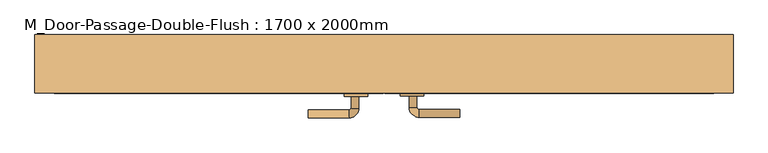
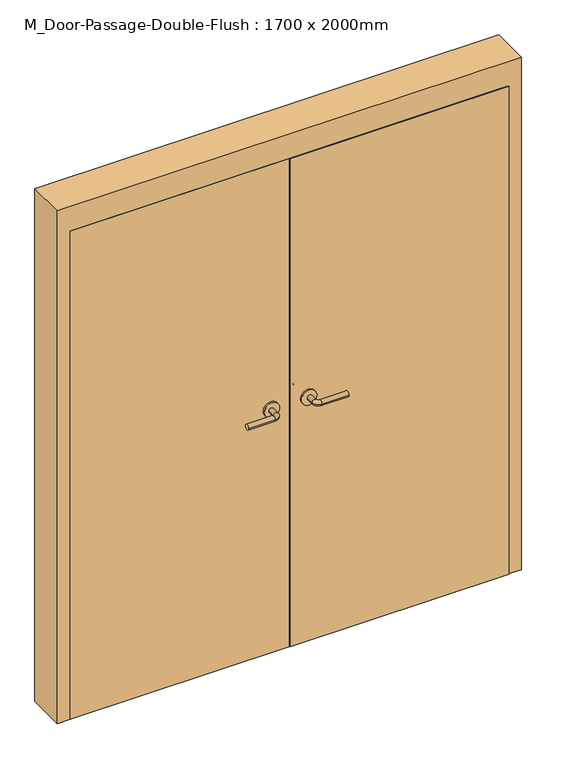
"""IFC4 building model written with IfcOpenShell, lengths in millimetres: door geometry, M_Door-Passage-Double-Flush : 1700 x 2000mm."""

from ifc_helpers import new_model, si_unit, point, frame, frame_2d, origin, origin_with_axes, place, context, project, spatial, polyline, circle_curve, ellipse_curve, trimmed, segment, composite_curve, outline, extrude, faceted_brep, source, transform, mapped, element, save
from ifc_brep_helpers import plane_surface, cylinder_surface, revolved_surface, advanced_brep


def m_door_passage_double_flush_1700_x_2000mm_96374c9b(model_context):
    return source(origin(), model_context, "Body", "SolidModel", [
        advanced_brep(
        [(-65.009375, -28.35, 1016.0), (-85.009375, -28.35, 1016.0), (-85.009375, 1.65, 1016.0), (-65.009375, 1.65, 1016.0), (-90.009375, 6.65, 1016.0), (-90.009375, 26.65, 1016.0), (-195.009375, 26.65, 1016.0), (-195.009375, 6.65, 1016.0)],
        [
            (0, 1, circle_curve(frame((-75.009375, -28.35, 1016.0), z_axis=(0.0, -1.0, 0.0), x_axis=(-1.0, 0.0, 0.0)), 10.0)),
            (1, 0, circle_curve(frame((-75.009375, -28.35, 1016.0), z_axis=(0.0, -1.0, 0.0), x_axis=(-1.0, 0.0, 0.0)), 10.0)),
            (1, 2),
            (2, 3, circle_curve(frame((-75.009375, 1.65, 1016.0), z_axis=(0.0, -1.0, 0.0), x_axis=(-1.0, 0.0, 0.0)), 10.0)),
            (3, 0),
            (3, 2, circle_curve(frame((-75.009375, 1.65, 1016.0), z_axis=(0.0, -1.0, 0.0), x_axis=(-1.0, 0.0, 0.0)), 10.0)),
            (4, 5, circle_curve(frame((-90.009375, 16.65, 1016.0), z_axis=(1.0, 0.0, 0.0), x_axis=(0.0, -1.0, 0.0)), 10.0)),
            (5, 3, circle_curve(frame((-90.009375, 1.65, 1016.0), z_axis=(0.0, 0.0, -1.0), x_axis=(1.0, 0.0, 0.0)), 25.0)),
            (2, 4, circle_curve(frame((-90.009375, 1.65, 1016.0), z_axis=(0.0, 0.0, 1.0), x_axis=(1.0, 0.0, 0.0)), 5.0)),
            (5, 4, circle_curve(frame((-90.009375, 16.65, 1016.0), z_axis=(1.0, 0.0, 0.0), x_axis=(0.0, -1.0, 0.0)), 10.0)),
            (6, 7, circle_curve(frame((-195.009375, 16.65, 1016.0), z_axis=(-1.0, 0.0, 0.0), x_axis=(0.0, -1.0, 0.0)), 10.0)),
            (7, 6, circle_curve(frame((-195.009375, 16.65, 1016.0), z_axis=(-1.0, 0.0, 0.0), x_axis=(0.0, -1.0, 0.0)), 10.0)),
            (4, 7),
            (6, 5),
        ],
        [
            plane_surface(frame((-75.009375, -28.35, 1016.0), z_axis=(0.0, -1.0, 0.0), x_axis=(0.0, 0.0, 1.0))),
            cylinder_surface(frame((-75.009375, -28.35, 1016.0), z_axis=(0.0, -1.0, 0.0), x_axis=(-1.0, 0.0, 0.0)), 10.0),
            revolved_surface(trimmed(ellipse_curve(frame((-75.009375, 1.65, 1016.0), z_axis=(0.0, 1.0, 0.0), x_axis=(-1.0, 0.0, 0.0)), 10.0, 10.0), [point((-65.009375, 1.65, 1016.0))], [point((-85.009375, 1.65, 1016.0))], True, "CARTESIAN"), (-90.009375, 1.65, 1016.0), (0.0, 0.0, -1.0)),
            revolved_surface(trimmed(ellipse_curve(frame((-75.009375, 1.65, 1016.0), z_axis=(0.0, 1.0, 0.0), x_axis=(-1.0, 0.0, 0.0)), 10.0, 10.0), [point((-85.009375, 1.65, 1016.0))], [point((-65.009375, 1.65, 1016.0))], True, "CARTESIAN"), (-90.009375, 1.65, 1016.0), (0.0, 0.0, -1.0)),
            plane_surface(frame((-195.009375, 16.65, 1016.0), z_axis=(-1.0, 0.0, 0.0), x_axis=(0.0, 0.0, 1.0))),
            cylinder_surface(frame((-90.009375, 16.65, 1016.0), z_axis=(1.0, 0.0, 0.0), x_axis=(0.0, -1.0, 0.0)), 10.0),
        ],
        [
            (0, [[1, 2]]),
            (1, [[3, 4, 5, -2]]),
            (1, [[-5, 6, -3, -1]]),
            (2, [[7, 8, -4, 9]]),
            (3, [[10, -9, -6, -8]]),
            (4, [[11, 12]]),
            (5, [[13, -11, 14, -7]]),
            (5, [[-14, -12, -13, -10]]),
        ],
    ),
        extrude(outline(composite_curve([segment(trimmed(circle_curve(frame_2d((1016.0, -72.509375)), 30.0), [point((1016.0, -42.509375))], [point((1016.0, -102.509375))], False, "CARTESIAN"), True, "CONTINUOUS"), segment(trimmed(circle_curve(frame_2d((1016.0, -72.509375)), 30.0), [point((1016.0, -102.509375))], [point((1016.0, -42.509375))], False, "CARTESIAN"), True, "CONTINUOUS")], self_intersect=False)), frame((0.0, -36.35, 0.0), z_axis=(0.0, 1.0, 0.0), x_axis=(0.0, 0.0, 1.0)), (0.0, 0.0, 1.0), 8.0),
        advanced_brep(
        [(-65.009375, -90.95, 1000.0), (-85.009375, -90.95, 1000.0), (-65.009375, -120.95, 1000.0), (-85.009375, -120.95, 1000.0), (-90.009375, -125.95, 1000.0), (-90.009375, -145.95, 1000.0), (-195.009375, -145.95, 1000.0), (-195.009375, -125.95, 1000.0)],
        [
            (0, 1, circle_curve(frame((-75.009375, -90.95, 1000.0), z_axis=(0.0, 1.0, 0.0), x_axis=(-1.0, 0.0, 0.0)), 10.0)),
            (1, 0, circle_curve(frame((-75.009375, -90.95, 1000.0), z_axis=(0.0, 1.0, 0.0), x_axis=(-1.0, 0.0, 0.0)), 10.0)),
            (0, 2),
            (2, 3, circle_curve(frame((-75.009375, -120.95, 1000.0), z_axis=(0.0, 1.0, 0.0), x_axis=(-1.0, 0.0, 0.0)), 10.0)),
            (3, 1),
            (3, 2, circle_curve(frame((-75.009375, -120.95, 1000.0), z_axis=(0.0, 1.0, 0.0), x_axis=(-1.0, 0.0, 0.0)), 10.0)),
            (4, 3, circle_curve(frame((-90.009375, -120.95, 1000.0), z_axis=(0.0, 0.0, 1.0), x_axis=(1.0, 0.0, 0.0)), 5.0)),
            (2, 5, circle_curve(frame((-90.009375, -120.95, 1000.0), z_axis=(0.0, 0.0, -1.0), x_axis=(1.0, 0.0, 0.0)), 25.0)),
            (5, 4, circle_curve(frame((-90.009375, -135.95, 1000.0), z_axis=(1.0, 0.0, 0.0), x_axis=(0.0, 1.0, 0.0)), 10.0)),
            (4, 5, circle_curve(frame((-90.009375, -135.95, 1000.0), z_axis=(1.0, 0.0, 0.0), x_axis=(0.0, 1.0, 0.0)), 10.0)),
            (6, 7, circle_curve(frame((-195.009375, -135.95, 1000.0), z_axis=(-1.0, 0.0, 0.0), x_axis=(0.0, 1.0, 0.0)), 10.0)),
            (7, 6, circle_curve(frame((-195.009375, -135.95, 1000.0), z_axis=(-1.0, 0.0, 0.0), x_axis=(0.0, 1.0, 0.0)), 10.0)),
            (5, 6),
            (7, 4),
        ],
        [
            plane_surface(frame((-75.009375, -90.95, 1000.0), z_axis=(0.0, 1.0, 0.0), x_axis=(0.0, 0.0, 1.0))),
            cylinder_surface(frame((-75.009375, -90.95, 1000.0), z_axis=(0.0, 1.0, 0.0), x_axis=(-1.0, 0.0, 0.0)), 10.0),
            revolved_surface(trimmed(ellipse_curve(frame((-75.009375, -120.95, 1000.0), z_axis=(0.0, 1.0, 0.0), x_axis=(-1.0, 0.0, 0.0)), 10.0, 10.0), [point((-65.009375, -120.95, 1000.0))], [point((-85.009375, -120.95, 1000.0))], True, "CARTESIAN"), (-90.009375, -120.95, 1000.0), (0.0, 0.0, -1.0)),
            revolved_surface(trimmed(ellipse_curve(frame((-75.009375, -120.95, 1000.0), z_axis=(0.0, 1.0, 0.0), x_axis=(-1.0, 0.0, 0.0)), 10.0, 10.0), [point((-85.009375, -120.95, 1000.0))], [point((-65.009375, -120.95, 1000.0))], True, "CARTESIAN"), (-90.009375, -120.95, 1000.0), (0.0, 0.0, -1.0)),
            plane_surface(frame((-195.009375, -135.95, 1000.0), z_axis=(-1.0, 0.0, 0.0), x_axis=(0.0, 0.0, 1.0))),
            cylinder_surface(frame((-90.009375, -135.95, 1000.0), z_axis=(1.0, 0.0, 0.0), x_axis=(0.0, 1.0, 0.0)), 10.0),
        ],
        [
            (0, [[1, 2]]),
            (1, [[-1, 3, 4, 5]]),
            (1, [[-2, -5, 6, -3]]),
            (2, [[7, -4, 8, 9]]),
            (3, [[-8, -6, -7, 10]]),
            (4, [[11, 12]]),
            (5, [[-9, 13, -12, 14]]),
            (5, [[-10, -14, -11, -13]]),
        ],
    ),
        extrude(outline(composite_curve([segment(trimmed(circle_curve(frame_2d((1000.0, -72.509375)), 30.0), [point((1000.0, -42.509375))], [point((1000.0, -102.509375))], False, "CARTESIAN"), True, "CONTINUOUS"), segment(trimmed(circle_curve(frame_2d((1000.0, -72.509375)), 30.0), [point((1000.0, -102.509375))], [point((1000.0, -42.509375))], False, "CARTESIAN"), True, "CONTINUOUS")], self_intersect=False)), frame((0.0, -90.95, 0.0), z_axis=(0.0, 1.0, 0.0), x_axis=(0.0, 0.0, 1.0)), (0.0, 0.0, 1.0), 8.0),
        advanced_brep(
        [(65.009375, -28.35, 1000.0), (85.009375, -28.35, 1000.0), (65.009375, 1.65, 1000.0), (85.009375, 1.65, 1000.0), (90.009375, 6.65, 1000.0), (90.009375, 26.65, 1000.0), (195.009375, 26.65, 1000.0), (195.009375, 6.65, 1000.0)],
        [
            (0, 1, circle_curve(frame((75.009375, -28.35, 1000.0), z_axis=(0.0, -1.0, 0.0), x_axis=(1.0, 0.0, 0.0)), 10.0)),
            (1, 0, circle_curve(frame((75.009375, -28.35, 1000.0), z_axis=(0.0, -1.0, 0.0), x_axis=(1.0, 0.0, 0.0)), 10.0)),
            (0, 2),
            (2, 3, circle_curve(frame((75.009375, 1.65, 1000.0), z_axis=(0.0, -1.0, 0.0), x_axis=(1.0, 0.0, 0.0)), 10.0)),
            (3, 1),
            (3, 2, circle_curve(frame((75.009375, 1.65, 1000.0), z_axis=(0.0, -1.0, 0.0), x_axis=(1.0, 0.0, 0.0)), 10.0)),
            (4, 3, circle_curve(frame((90.009375, 1.65, 1000.0), z_axis=(0.0, 0.0, 1.0), x_axis=(-1.0, 0.0, 0.0)), 5.0)),
            (2, 5, circle_curve(frame((90.009375, 1.65, 1000.0), z_axis=(0.0, 0.0, -1.0), x_axis=(-1.0, 0.0, 0.0)), 25.0)),
            (5, 4, circle_curve(frame((90.009375, 16.65, 1000.0), z_axis=(-1.0, 0.0, 0.0), x_axis=(0.0, -1.0, 0.0)), 10.0)),
            (4, 5, circle_curve(frame((90.009375, 16.65, 1000.0), z_axis=(-1.0, 0.0, 0.0), x_axis=(0.0, -1.0, 0.0)), 10.0)),
            (6, 7, circle_curve(frame((195.009375, 16.65, 1000.0), z_axis=(1.0, 0.0, 0.0), x_axis=(0.0, -1.0, 0.0)), 10.0)),
            (7, 6, circle_curve(frame((195.009375, 16.65, 1000.0), z_axis=(1.0, 0.0, 0.0), x_axis=(0.0, -1.0, 0.0)), 10.0)),
            (5, 6),
            (7, 4),
        ],
        [
            plane_surface(frame((75.009375, -28.35, 1000.0), z_axis=(0.0, -1.0, 0.0), x_axis=(0.0, 0.0, 1.0))),
            cylinder_surface(frame((75.009375, -28.35, 1000.0), z_axis=(0.0, -1.0, 0.0), x_axis=(1.0, 0.0, 0.0)), 10.0),
            revolved_surface(trimmed(ellipse_curve(frame((75.009375, 1.65, 1000.0), z_axis=(0.0, -1.0, 0.0), x_axis=(1.0, 0.0, 0.0)), 10.0, 10.0), [point((65.009375, 1.65, 1000.0))], [point((85.009375, 1.65, 1000.0))], True, "CARTESIAN"), (90.009375, 1.65, 1000.0), (0.0, 0.0, -1.0)),
            revolved_surface(trimmed(ellipse_curve(frame((75.009375, 1.65, 1000.0), z_axis=(0.0, -1.0, 0.0), x_axis=(1.0, 0.0, 0.0)), 10.0, 10.0), [point((85.009375, 1.65, 1000.0))], [point((65.009375, 1.65, 1000.0))], True, "CARTESIAN"), (90.009375, 1.65, 1000.0), (0.0, 0.0, -1.0)),
            plane_surface(frame((195.009375, 16.65, 1000.0), z_axis=(1.0, 0.0, 0.0), x_axis=(0.0, 0.0, 1.0))),
            cylinder_surface(frame((90.009375, 16.65, 1000.0), z_axis=(-1.0, 0.0, 0.0), x_axis=(0.0, -1.0, 0.0)), 10.0),
        ],
        [
            (0, [[1, 2]]),
            (1, [[-1, 3, 4, 5]]),
            (1, [[-2, -5, 6, -3]]),
            (2, [[7, -4, 8, 9]]),
            (3, [[-8, -6, -7, 10]]),
            (4, [[11, 12]]),
            (5, [[-9, 13, -12, 14]]),
            (5, [[-10, -14, -11, -13]]),
        ],
    ),
        extrude(outline(composite_curve([segment(trimmed(circle_curve(frame_2d((1000.0, 72.509375)), 30.0), [point((1000.0, 42.509375))], [point((1000.0, 102.509375))], False, "CARTESIAN"), True, "CONTINUOUS"), segment(trimmed(circle_curve(frame_2d((1000.0, 72.509375)), 30.0), [point((1000.0, 102.509375))], [point((1000.0, 42.509375))], False, "CARTESIAN"), True, "CONTINUOUS")], self_intersect=False)), frame((0.0, -36.35, 0.0), z_axis=(0.0, 1.0, 0.0), x_axis=(0.0, 0.0, 1.0)), (0.0, 0.0, 1.0), 8.0),
        advanced_brep(
        [(65.009375, -89.35, 1000.0), (85.009375, -89.35, 1000.0), (85.009375, -119.35, 1000.0), (65.009375, -119.35, 1000.0), (90.009375, -124.35, 1000.0), (90.009375, -144.35, 1000.0), (195.009375, -144.35, 1000.0), (195.009375, -124.35, 1000.0)],
        [
            (0, 1, circle_curve(frame((75.009375, -89.35, 1000.0), z_axis=(0.0, 1.0, 0.0), x_axis=(1.0, 0.0, 0.0)), 10.0)),
            (1, 0, circle_curve(frame((75.009375, -89.35, 1000.0), z_axis=(0.0, 1.0, 0.0), x_axis=(1.0, 0.0, 0.0)), 10.0)),
            (1, 2),
            (2, 3, circle_curve(frame((75.009375, -119.35, 1000.0), z_axis=(0.0, 1.0, 0.0), x_axis=(1.0, 0.0, 0.0)), 10.0)),
            (3, 0),
            (3, 2, circle_curve(frame((75.009375, -119.35, 1000.0), z_axis=(0.0, 1.0, 0.0), x_axis=(1.0, 0.0, 0.0)), 10.0)),
            (4, 5, circle_curve(frame((90.009375, -134.35, 1000.0), z_axis=(-1.0, 0.0, 0.0), x_axis=(0.0, 1.0, 0.0)), 10.0)),
            (5, 3, circle_curve(frame((90.009375, -119.35, 1000.0), z_axis=(0.0, 0.0, -1.0), x_axis=(-1.0, 0.0, 0.0)), 25.0)),
            (2, 4, circle_curve(frame((90.009375, -119.35, 1000.0), z_axis=(0.0, 0.0, 1.0), x_axis=(-1.0, 0.0, 0.0)), 5.0)),
            (5, 4, circle_curve(frame((90.009375, -134.35, 1000.0), z_axis=(-1.0, 0.0, 0.0), x_axis=(0.0, 1.0, 0.0)), 10.0)),
            (6, 7, circle_curve(frame((195.009375, -134.35, 1000.0), z_axis=(1.0, 0.0, 0.0), x_axis=(0.0, 1.0, 0.0)), 10.0)),
            (7, 6, circle_curve(frame((195.009375, -134.35, 1000.0), z_axis=(1.0, 0.0, 0.0), x_axis=(0.0, 1.0, 0.0)), 10.0)),
            (4, 7),
            (6, 5),
        ],
        [
            plane_surface(frame((75.009375, -89.35, 1000.0), z_axis=(0.0, 1.0, 0.0), x_axis=(0.0, 0.0, 1.0))),
            cylinder_surface(frame((75.009375, -89.35, 1000.0), z_axis=(0.0, 1.0, 0.0), x_axis=(1.0, 0.0, 0.0)), 10.0),
            revolved_surface(trimmed(ellipse_curve(frame((75.009375, -119.35, 1000.0), z_axis=(0.0, -1.0, 0.0), x_axis=(1.0, 0.0, 0.0)), 10.0, 10.0), [point((65.009375, -119.35, 1000.0))], [point((85.009375, -119.35, 1000.0))], True, "CARTESIAN"), (90.009375, -119.35, 1000.0), (0.0, 0.0, -1.0)),
            revolved_surface(trimmed(ellipse_curve(frame((75.009375, -119.35, 1000.0), z_axis=(0.0, -1.0, 0.0), x_axis=(1.0, 0.0, 0.0)), 10.0, 10.0), [point((85.009375, -119.35, 1000.0))], [point((65.009375, -119.35, 1000.0))], True, "CARTESIAN"), (90.009375, -119.35, 1000.0), (0.0, 0.0, -1.0)),
            plane_surface(frame((195.009375, -134.35, 1000.0), z_axis=(1.0, 0.0, 0.0), x_axis=(0.0, 0.0, 1.0))),
            cylinder_surface(frame((90.009375, -134.35, 1000.0), z_axis=(-1.0, 0.0, 0.0), x_axis=(0.0, 1.0, 0.0)), 10.0),
        ],
        [
            (0, [[1, 2]]),
            (1, [[3, 4, 5, -2]]),
            (1, [[-5, 6, -3, -1]]),
            (2, [[7, 8, -4, 9]]),
            (3, [[10, -9, -6, -8]]),
            (4, [[11, 12]]),
            (5, [[13, -11, 14, -7]]),
            (5, [[-14, -12, -13, -10]]),
        ],
    ),
        extrude(outline(composite_curve([segment(trimmed(circle_curve(frame_2d((1000.0, 72.509375)), 30.0), [point((1000.0, 42.509375))], [point((1000.0, 102.509375))], False, "CARTESIAN"), True, "CONTINUOUS"), segment(trimmed(circle_curve(frame_2d((1000.0, 72.509375)), 30.0), [point((1000.0, 102.509375))], [point((1000.0, 42.509375))], False, "CARTESIAN"), True, "CONTINUOUS")], self_intersect=False)), frame((0.0, -89.35, 0.0), z_axis=(0.0, 1.0, 0.0), x_axis=(0.0, 0.0, 1.0)), (0.0, 0.0, 1.0), 8.0),
        extrude(outline(polyline([(850.0, -36.35), (850.0, -82.95), (1.5875, -82.95), (1.5875, -36.35), (850.0, -36.35)])), origin_with_axes(), (0.0, 0.0, 1.0), 2000.0),
        extrude(outline(polyline([(-1.5875, -36.35), (-1.5875, -82.95), (-850.0, -82.95), (-850.0, -36.35), (-1.5875, -36.35)])), origin_with_axes(), (0.0, 0.0, 1.0), 2000.0),
        faceted_brep([(850.0, -31.5875, 0.0), (834.125, -31.5875, 0.0), (834.125, 19.4375, 0.0), (850.0, 19.4375, 0.0), (850.0, 68.65, 0.0), (900.0, 68.65, 0.0), (900.0, -81.35, 0.0), (850.0, -81.35, 0.0), (850.0, -81.35, 2000.0), (850.0, -31.5875, 2000.0), (900.0, -81.35, 2100.0), (-900.0, -81.35, 2100.0), (-900.0, -81.35, 0.0), (-850.0, -81.35, 0.0), (-850.0, -81.35, 2000.0), (900.0, 68.65, 2100.0), (850.0, 68.65, 2000.0), (-850.0, 68.65, 2000.0), (-850.0, 68.65, 0.0), (-900.0, 68.65, 0.0), (-900.0, 68.65, 2100.0), (850.0, 19.4375, 2000.0), (834.125, 19.4375, 1984.125), (-834.125, 19.4375, 1984.125), (-834.125, 19.4375, 0.0), (-850.0, 19.4375, 0.0), (-850.0, 19.4375, 2000.0), (834.125, -31.5875, 1984.125), (-850.0, -31.5875, 2000.0), (-850.0, -31.5875, 0.0), (-834.125, -31.5875, 0.0), (-834.125, -31.5875, 1984.125)], [[[0, 1, 2, 3, 4, 5, 6, 7]], [[7, 8, 9, 0]], [[6, 10, 11, 12, 13, 14, 8, 7]], [[5, 15, 10, 6]], [[4, 16, 17, 18, 19, 20, 15, 5]], [[3, 21, 16, 4]], [[2, 22, 23, 24, 25, 26, 21, 3]], [[1, 27, 22, 2]], [[0, 9, 28, 29, 30, 31, 27, 1]], [[8, 14, 28, 9]], [[16, 21, 26, 17]], [[22, 27, 31, 23]], [[12, 19, 18, 25, 24, 30, 29, 13]], [[13, 29, 28, 14]], [[11, 20, 19, 12]], [[17, 26, 25, 18]], [[23, 31, 30, 24]], [[15, 20, 11, 10]]]),
    ])


if __name__ == "__main__":
    model = new_model("IFC4")
    model_context = context("Model", 3, world=origin())
    ifc_project = project(units=[si_unit("LENGTHUNIT", "METRE", prefix="MILLI")], contexts=[model_context])
    site = spatial("IfcSite", under=ifc_project)
    building = spatial("IfcBuilding", under=site)
    placement = place(None, origin())
    m_door_passage_double_flush_1700_x_2000mm_shape = m_door_passage_double_flush_1700_x_2000mm_96374c9b(model_context)
    element("IfcDoor", 1, ObjectType="M_Door-Passage-Double-Flush : 1700 x 2000mm", at=placement, inside=building, context=model_context, shape_type="MappedRepresentation", body=[
        mapped(m_door_passage_double_flush_1700_x_2000mm_shape, transform((0.0, 0.0, 0.0), x_axis=(1.0, 0.0, 0.0), y_axis=(0.0, 1.0, 0.0), z_axis=(0.0, 0.0, 1.0))),
    ])
    save(model, "model.ifc")

# Revit data of these elements
# Type "M_Door-Passage-Double-Flush : 1700 x 2000mm"
#   Type Mark = "31"
#   Analytic Construction = "Metal"
#   Thickness = 45 mm
#   Thermal Resistance (R) = 0.270118 (m²·K)/W
#   Swing Angle [instance default] = 90.00°
#   Strike Height = 1000 mm
#   SinglePanelWidth = 850 mm
#   Rough Width [instance default] = 1800 mm
#   Rough Height [instance default] = 2100 mm
#   MFOpeningHeight [instance default] = 100 mm
#   MFOpeningWidth [instance default] = 100 mm
#   Inset Calculate [instance default] = 105 mm
#   Masonry Inset [instance default] = 25 mm
#   Height = 2000 mm
#   Width = 1700 mm
#   Heat Transfer Coefficient (U) = 3.70223 W/(m²·K)
#   Masonry Frame Depth = 150 mm
#   Masonry Frame [instance default] = yes
#   Function = 1
#   Dry Wall Frame [instance default] = no
#   Panel Material = Metal Door - Brindle
#   Frame Material = Metal - Painted - Grey
#   Door Handle Material = Aluminum
#   Visual Light Transmittance = 0
#   Solar Heat Gain Coefficient = 0
#   Wall Closure = (empty or 0)
# Element 1 (IfcDoor, "M_Door-Passage-Double-Flush : 1700 x 2000mm")
#   Materials on its faces: "Aluminum", "Metal - Painted - Grey", "Metal Door - Brindle"
# Materials
#   "Metal Door - Brindle": class "Paint", colour RGB 164 133 98, transparency 0
#   "Metal - Painted - Grey": class "Paint", colour RGB 104 104 104, transparency 0
#   "Aluminum": class "Metal", colour RGB 244 245 246, transparency 0, Description = "Aluminum 6061", Cost = 0
